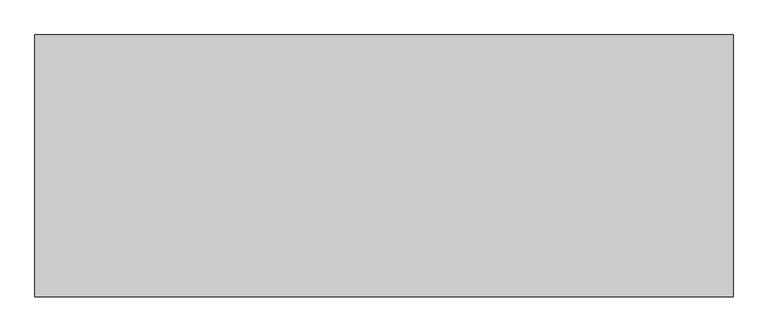
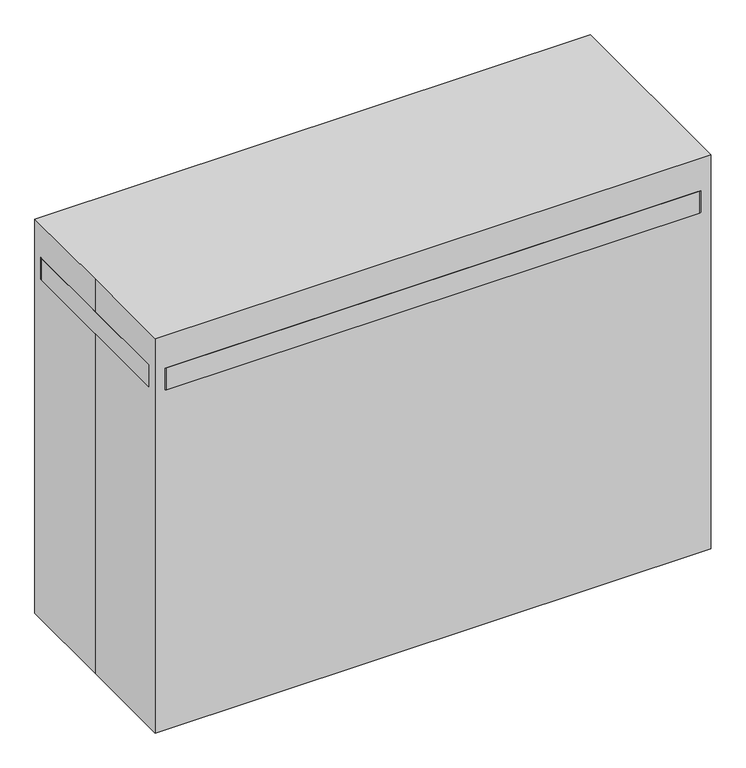
"""IFC4 building model written with IfcOpenShell, lengths in millimetres: proxy geometry, TB018 - Backtable : TB018 - Backtable."""

import ifcopenshell
import ifcopenshell.guid

model = None  # the IFC model being written
_history = None  # IfcOwnerHistory: only IFC2X3 demands one
_inside = {}  # id of a spatial element -> (the spatial element, [elements in it])
_under = {}  # id of a project, library or spatial element -> (it, [spatial elements below it])
_declared = {}  # id of a project -> (the project, [libraries it declares])
_typed = {}  # id of a type object -> (the type object, [elements of that type])
_made_of = {}  # id of a material, layer set ... -> (it, [elements and type objects made of it])


def new_model(schema):
    """Start an empty IFC model of exactly this schema.

    Asked for "IFC4X3", IfcOpenShell would pick the latest addendum, in which some entities
    have other attributes; the version numbers below select the first issue.
    IFC2X3 requires an IfcOwnerHistory on every rooted entity: one is made here for all.
    """
    global model, _history
    if schema == "IFC4X3":
        model = ifcopenshell.file(schema_version=(4, 3, 0, 0))
    else:
        model = ifcopenshell.file(schema=schema)
    _inside.clear()
    _under.clear()
    _declared.clear()
    _typed.clear()
    _made_of.clear()
    _history = None
    if model.schema == "IFC2X3":
        org = make("IfcOrganization", Name="unknown")
        user = make(
            "IfcPersonAndOrganization",
            ThePerson=make("IfcPerson", FamilyName="unknown"),
            TheOrganization=org,
        )
        app = make(
            "IfcApplication",
            ApplicationDeveloper=org,
            Version="unknown",
            ApplicationFullName="unknown",
            ApplicationIdentifier="unknown",
        )
        _history = make(
            "IfcOwnerHistory",
            OwningUser=user,
            OwningApplication=app,
            ChangeAction="ADDED",
            CreationDate=0,
        )
    return model


def make(cls, **values):
    """One entity of the class cls with the attributes given. An attribute that is None is left unset."""
    return model.create_entity(
        cls, **{name: value for name, value in values.items() if value is not None}
    )


def rooted(cls, **values):
    """An entity with a GlobalId (a new one), such as an element, a storey or a relation."""
    return make(cls, GlobalId=ifcopenshell.guid.new(), OwnerHistory=_history, **values)


def si_unit(unit_type, name, prefix=None):
    """IfcSIUnit, for example si_unit("LENGTHUNIT", "METRE", prefix="MILLI")."""
    return make("IfcSIUnit", UnitType=unit_type, Prefix=prefix, Name=name)


def assignment(units):
    """IfcUnitAssignment: the units of a project."""
    return None if units is None else make("IfcUnitAssignment", Units=units)


def point(xyz):
    """IfcCartesianPoint."""
    return None if xyz is None else make("IfcCartesianPoint", Coordinates=xyz)


def direction(xyz):
    """IfcDirection."""
    return None if xyz is None else make("IfcDirection", DirectionRatios=xyz)


def frame(location, z_axis=None, x_axis=None):
    """IfcAxis2Placement3D, a coordinate frame: its origin and axes. An axis left out is left unset."""
    return make(
        "IfcAxis2Placement3D",
        Location=point(location),
        Axis=direction(z_axis),
        RefDirection=direction(x_axis),
    )


def frame_2d(location, x_axis=None):
    """IfcAxis2Placement2D, a coordinate frame in the plane: its origin and x axis."""
    return make(
        "IfcAxis2Placement2D", Location=point(location), RefDirection=direction(x_axis)
    )


def origin():
    """The frame at (0, 0, 0) with its axes left unset."""
    return frame((0.0, 0.0, 0.0))


def origin_with_axes():
    """The frame at (0, 0, 0) with the z axis (0, 0, 1) and the x axis (1, 0, 0) written out."""
    return frame((0.0, 0.0, 0.0), z_axis=(0.0, 0.0, 1.0), x_axis=(1.0, 0.0, 0.0))


def place(relative_to, where):
    """IfcLocalPlacement: puts the frame where relative to a parent placement (None: the world)."""
    return make(
        "IfcLocalPlacement", PlacementRelTo=relative_to, RelativePlacement=where
    )


def context(
    kind, dimensions, precision=None, world=None, true_north=None, identifier=None
):
    """IfcGeometricRepresentationContext, for example the 3D "Model" context."""
    return make(
        "IfcGeometricRepresentationContext",
        ContextIdentifier=identifier,
        ContextType=kind,
        CoordinateSpaceDimension=dimensions,
        Precision=precision,
        WorldCoordinateSystem=world,
        TrueNorth=true_north,
    )


def project(units=None, contexts=None):
    """IfcProject with its units and contexts."""
    return rooted(
        "IfcProject",
        Name="project",
        RepresentationContexts=contexts,
        UnitsInContext=assignment(units),
    )


def spatial(cls, under=None, at=None, **own):
    """A site, building, storey or space (cls), placed at a placement, below another one or the project."""
    s = rooted(cls, ObjectPlacement=at, **own)
    if under is not None:
        _under.setdefault(under.id(), (under, []))[1].append(s)
    return s


def polyline(points):
    """IfcPolyline through the points."""
    return make("IfcPolyline", Points=[point(p) for p in points])


def circle_curve(where, radius):
    """IfcCircle in the frame where."""
    return make("IfcCircle", Position=where, Radius=radius)


def trimmed(basis, trim1, trim2, sense, master):
    """IfcTrimmedCurve: the piece of a basis curve between two trims."""
    return make(
        "IfcTrimmedCurve",
        BasisCurve=basis,
        Trim1=trim1,
        Trim2=trim2,
        SenseAgreement=sense,
        MasterRepresentation=master,
    )


def segment(curve, same_sense, transition):
    """IfcCompositeCurveSegment."""
    return make(
        "IfcCompositeCurveSegment",
        Transition=transition,
        SameSense=same_sense,
        ParentCurve=curve,
    )


def composite_curve(segments, self_intersect=None):
    """IfcCompositeCurve: segments joined end to end."""
    return make("IfcCompositeCurve", Segments=segments, SelfIntersect=self_intersect)


def outline(outer, holes=None, kind="AREA"):
    """IfcArbitraryClosedProfileDef: a profile drawn as a closed curve; with holes, ...WithVoids."""
    if holes is None:
        return make("IfcArbitraryClosedProfileDef", ProfileType=kind, OuterCurve=outer)
    return make(
        "IfcArbitraryProfileDefWithVoids",
        ProfileType=kind,
        OuterCurve=outer,
        InnerCurves=holes,
    )


def extrude(swept, where, along, depth):
    """IfcExtrudedAreaSolid: the profile swept, set in the frame where, extruded along a direction by depth."""
    return make(
        "IfcExtrudedAreaSolid",
        SweptArea=swept,
        Position=where,
        ExtrudedDirection=direction(along),
        Depth=depth,
    )


def shape(context_of_items, identifier, shape_type, items):
    """IfcShapeRepresentation: the items that make up one representation, for example the "Body"."""
    return make(
        "IfcShapeRepresentation",
        ContextOfItems=context_of_items,
        RepresentationIdentifier=identifier,
        RepresentationType=shape_type,
        Items=items,
    )


def source(mapping_origin, context_of_items, identifier, shape_type, items):
    """IfcRepresentationMap: a shape defined once, which mapped items show again and again."""
    return make(
        "IfcRepresentationMap",
        MappingOrigin=mapping_origin,
        MappedRepresentation=shape(context_of_items, identifier, shape_type, items),
    )


def transform(
    local_origin,
    x_axis=None,
    y_axis=None,
    z_axis=None,
    scale=None,
    scale2=None,
    scale3=None,
    uniform=True,
):
    """IfcCartesianTransformationOperator3D, or its non-uniform kind. x_axis, y_axis, z_axis: its Axis1, 2, 3."""
    if uniform:
        return make(
            "IfcCartesianTransformationOperator3D",
            Axis1=direction(x_axis),
            Axis2=direction(y_axis),
            LocalOrigin=point(local_origin),
            Scale=scale,
            Axis3=direction(z_axis),
        )
    return make(
        "IfcCartesianTransformationOperator3DnonUniform",
        Axis1=direction(x_axis),
        Axis2=direction(y_axis),
        LocalOrigin=point(local_origin),
        Scale=scale,
        Axis3=direction(z_axis),
        Scale2=scale2,
        Scale3=scale3,
    )


def mapped(mapping_source, mapping_target):
    """IfcMappedItem: shows the shape of a source again, moved by a transform."""
    return make(
        "IfcMappedItem", MappingSource=mapping_source, MappingTarget=mapping_target
    )


def made_of(thing, what):
    """Note that an element or type object is made of a material, layer set ...; save() writes the relation."""
    if what is not None:
        _made_of.setdefault(what.id(), (what, []))[1].append(thing)
    return thing


def element(
    cls,
    number,
    at=None,
    inside=None,
    cuts=None,
    type_object=None,
    material=None,
    context=None,
    identifier="Body",
    shape_type=None,
    held_by="IfcProductDefinitionShape",
    body=None,
    shapes=None,
    **own,
):
    """One element of the class cls, such as IfcWall. Its Tag is "e" and its number.

    at: its placement. inside: the storey or other place that contains it. cuts: it is an
    opening in that element (IfcRelVoidsElement). A single representation is given by context,
    identifier, shape_type and body (its items); several are given by shapes. held_by: the class
    of the entity that holds the representations. save() writes the other relations.
    """
    e = rooted(cls, Tag="e%d" % number, ObjectPlacement=at, **own)
    if body is not None:
        shapes = [shape(context, identifier, shape_type, body)]
    if shapes is not None:
        e.Representation = make(held_by, Representations=shapes)
    if inside is not None:
        _inside.setdefault(inside.id(), (inside, []))[1].append(e)
    if cuts is not None:
        rooted(
            "IfcRelVoidsElement", RelatingBuildingElement=cuts, RelatedOpeningElement=e
        )
    if type_object is not None:
        _typed.setdefault(type_object.id(), (type_object, []))[1].append(e)
    return made_of(e, material)


def aggregate(whole, parts):
    """IfcRelAggregates: a whole, such as a stair, and the parts it consists of."""
    return rooted("IfcRelAggregates", RelatingObject=whole, RelatedObjects=parts)


def save(model, path):
    """Write the relations noted so far, then the file.

    IfcRelAggregates (storeys below a building ...), IfcRelContainedInSpatialStructure (elements
    in a storey), IfcRelDefinesByType, IfcRelAssociatesMaterial and IfcRelDeclares: one each for
    every whole, place, type object, material and project.
    """
    for whole, parts in _under.values():
        aggregate(whole, parts)
    for where, things in _inside.values():
        rooted(
            "IfcRelContainedInSpatialStructure",
            RelatedElements=things,
            RelatingStructure=where,
        )
    for kind, things in _typed.values():
        rooted("IfcRelDefinesByType", RelatedObjects=things, RelatingType=kind)
    for what, things in _made_of.values():
        rooted("IfcRelAssociatesMaterial", RelatedObjects=things, RelatingMaterial=what)
    for by, libraries in _declared.values():
        rooted("IfcRelDeclares", RelatingContext=by, RelatedDefinitions=libraries)
    model.write(path)


def specialty_equipment_5ab2001b(model_context):
    return source(origin(), model_context, "Body", "SweptSolid", [
        extrude(outline(composite_curve([segment(trimmed(circle_curve(frame_2d((584.2, 203.2)), 25.4), [point((584.2, 228.6))], [point((609.6, 203.2))], False, "CARTESIAN"), True, "CONTINUOUS"), segment(polyline([(609.6, 203.2), (609.6, -203.2)]), True, "CONTINUOUS"), segment(trimmed(circle_curve(frame_2d((584.2, -203.2)), 25.4), [point((609.6, -203.2))], [point((584.2, -228.6))], False, "CARTESIAN"), True, "CONTINUOUS"), segment(polyline([(584.2, -228.6), (-584.2, -228.6)]), True, "CONTINUOUS"), segment(trimmed(circle_curve(frame_2d((-584.2, -203.2)), 25.4), [point((-584.2, -228.6))], [point((-609.6, -203.2))], False, "CARTESIAN"), True, "CONTINUOUS"), segment(polyline([(-609.6, -203.2), (-609.6, 203.2)]), True, "CONTINUOUS"), segment(trimmed(circle_curve(frame_2d((-584.2, 203.2)), 25.4), [point((-609.6, 203.2))], [point((-584.2, 228.6))], False, "CARTESIAN"), True, "CONTINUOUS"), segment(polyline([(-584.2, 228.6), (584.2, 228.6)]), True, "CONTINUOUS")], self_intersect=False)), frame((0.0, 0.0, 787.4), z_axis=(0.0, 0.0, 1.0), x_axis=(1.0, 0.0, 0.0)), (0.0, 0.0, 1.0), 50.8),
        extrude(outline(composite_curve([segment(trimmed(circle_curve(frame_2d((-533.4, 152.4)), 38.1), [point((-571.5, 152.4))], [point((-495.3, 152.4))], False, "CARTESIAN"), True, "CONTINUOUS"), segment(trimmed(circle_curve(frame_2d((-533.4, 152.4)), 38.1), [point((-495.3, 152.4))], [point((-571.5, 152.4))], False, "CARTESIAN"), True, "CONTINUOUS")], self_intersect=False)), origin_with_axes(), (0.0, 0.0, 1.0), 787.4),
        extrude(outline(composite_curve([segment(trimmed(circle_curve(frame_2d((533.4, 152.4)), 38.1), [point((495.3, 152.4))], [point((571.5, 152.4))], False, "CARTESIAN"), True, "CONTINUOUS"), segment(trimmed(circle_curve(frame_2d((533.4, 152.4)), 38.1), [point((571.5, 152.4))], [point((495.3, 152.4))], False, "CARTESIAN"), True, "CONTINUOUS")], self_intersect=False)), origin_with_axes(), (0.0, 0.0, 1.0), 787.4),
        extrude(outline(composite_curve([segment(trimmed(circle_curve(frame_2d((-533.4, -152.4)), 38.1), [point((-571.5, -152.4))], [point((-495.3, -152.4))], False, "CARTESIAN"), True, "CONTINUOUS"), segment(trimmed(circle_curve(frame_2d((-533.4, -152.4)), 38.1), [point((-495.3, -152.4))], [point((-571.5, -152.4))], False, "CARTESIAN"), True, "CONTINUOUS")], self_intersect=False)), origin_with_axes(), (0.0, 0.0, 1.0), 787.4),
        extrude(outline(composite_curve([segment(trimmed(circle_curve(frame_2d((533.4, -152.4)), 38.1), [point((495.3, -152.4))], [point((571.5, -152.4))], False, "CARTESIAN"), True, "CONTINUOUS"), segment(trimmed(circle_curve(frame_2d((533.4, -152.4)), 38.1), [point((571.5, -152.4))], [point((495.3, -152.4))], False, "CARTESIAN"), True, "CONTINUOUS")], self_intersect=False)), origin_with_axes(), (0.0, 0.0, 1.0), 787.4),
        extrude(outline(polyline([(-609.6, 228.6), (609.6, 228.6), (609.6, -228.6), (-609.6, -228.6), (-609.6, 0.0), (-609.6, 228.6)])), origin_with_axes(), (0.0, 0.0, 1.0), 914.4),
    ])


if __name__ == "__main__":
    model = new_model("IFC4")
    model_context = context("Model", 3, world=origin())
    ifc_project = project(units=[si_unit("LENGTHUNIT", "METRE", prefix="MILLI")], contexts=[model_context])
    site = spatial("IfcSite", under=ifc_project)
    building = spatial("IfcBuilding", under=site)
    placement = place(None, origin())
    specialty_equipment_shape = specialty_equipment_5ab2001b(model_context)
    element("IfcBuildingElementProxy", 1, Name="TB018 - Backtable : TB018 - Backtable", ObjectType="TB018 - Backtable : TB018 - Backtable", at=placement, inside=building, context=model_context, shape_type="MappedRepresentation", body=[
        mapped(specialty_equipment_shape, transform((0.0, 0.0, 0.0), x_axis=(1.0, 0.0, 0.0), y_axis=(0.0, 1.0, 0.0), z_axis=(0.0, 0.0, 1.0))),
    ])
    save(model, "model.ifc")

# Revit data of these elements
# Type "TB018 - Backtable : TB018 - Backtable"
#   Watts2 = "0"
#   Watts1 = "0"
#   Unit_Issue = "EA"
#   UTIL_6_Misc = "-"
#   UTIL_5_NonMedGas = "-"
#   UTIL_4_MiscGas = "-"
#   UTIL_3_MedGas = "-"
#   UTIL_2_Elec = "-"
#   UTIL_1_WaterDrain = "-"
#   Nomenclature = "Backtable"
#   NSN = ""
#   Location [instance default] = ""
#   JSN = "TB018"
#   Fund_Source_VA = "-"
#   Fund_Source_Navy = "-"
#   Fund_Source_Army = "-"
#   Fund_Source_AF = "-"
#   ELEC_Volts2 = "0"
#   ELEC_Volts1 = "0"
#   ELEC_Phase2 = "0"
#   ELEC_Phase1 = "0"
#   ELEC_HertzSwitch = "0"
#   ELEC_HertzDependent = "0"
#   ELEC_Hertz = "0"
#   ELEC_Amps2 = "0"
#   ELEC_Amps1 = "0"
#   DetailDescription = ""
#   CAT_VA = "C"
#   CAT_Navy = "C"
#   CAT_IHS = "-"
#   CAT_Army = "C"
#   CAT_AF = "C"
#   BTUperhour = "0"
#   Weight_IP = 0
#   DIM_Width_IP = 4' - 0"
#   DIM_Height_IP = 3' - 0"
#   DIM_Depth_IP = 1' - 6"
# Element 1 (IfcBuildingElementProxy, "TB018 - Backtable : TB018 - Backtable")
#   Materials on its faces: "EquipSpace"
# Materials
#   "EquipSpace": class "Unassigned", colour RGB 221 217 195, transparency 0.5
